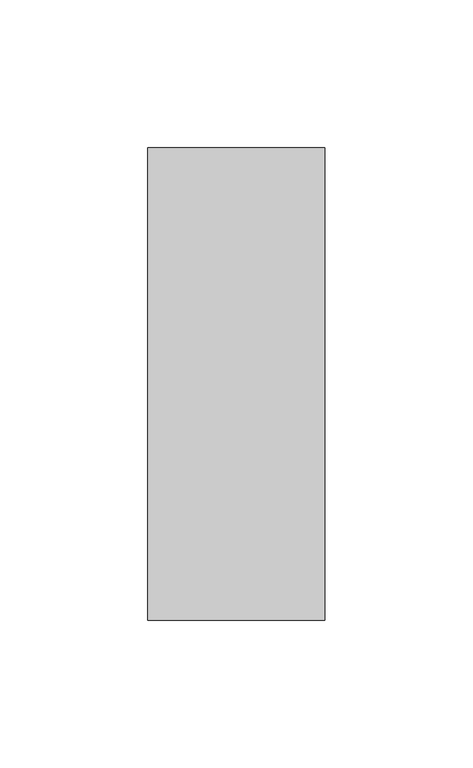
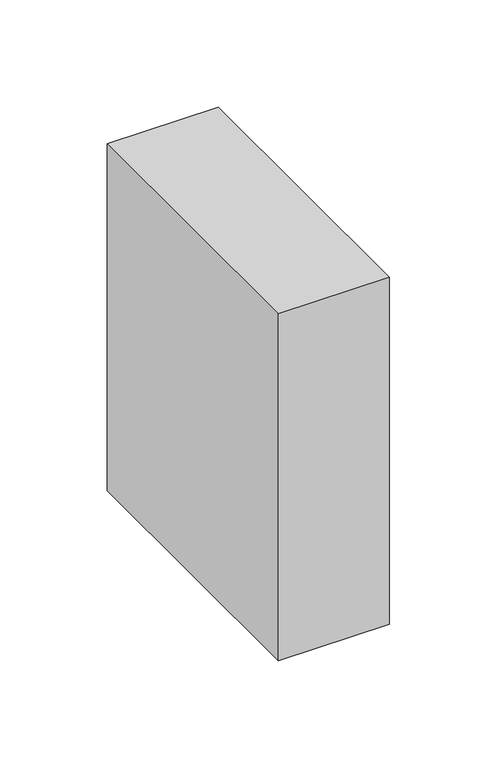
"""IFC4 building model written with IfcOpenShell, lengths in millimetres: column geometry, Madeira de lei-Coluna : Pontalete 6X16cm."""

import ifcopenshell
import ifcopenshell.guid

model = None  # the IFC model being written
_history = None  # IfcOwnerHistory: only IFC2X3 demands one
_inside = {}  # id of a spatial element -> (the spatial element, [elements in it])
_under = {}  # id of a project, library or spatial element -> (it, [spatial elements below it])
_declared = {}  # id of a project -> (the project, [libraries it declares])
_typed = {}  # id of a type object -> (the type object, [elements of that type])
_made_of = {}  # id of a material, layer set ... -> (it, [elements and type objects made of it])


def new_model(schema):
    """Start an empty IFC model of exactly this schema.

    Asked for "IFC4X3", IfcOpenShell would pick the latest addendum, in which some entities
    have other attributes; the version numbers below select the first issue.
    IFC2X3 requires an IfcOwnerHistory on every rooted entity: one is made here for all.
    """
    global model, _history
    if schema == "IFC4X3":
        model = ifcopenshell.file(schema_version=(4, 3, 0, 0))
    else:
        model = ifcopenshell.file(schema=schema)
    _inside.clear()
    _under.clear()
    _declared.clear()
    _typed.clear()
    _made_of.clear()
    _history = None
    if model.schema == "IFC2X3":
        org = make("IfcOrganization", Name="unknown")
        user = make(
            "IfcPersonAndOrganization",
            ThePerson=make("IfcPerson", FamilyName="unknown"),
            TheOrganization=org,
        )
        app = make(
            "IfcApplication",
            ApplicationDeveloper=org,
            Version="unknown",
            ApplicationFullName="unknown",
            ApplicationIdentifier="unknown",
        )
        _history = make(
            "IfcOwnerHistory",
            OwningUser=user,
            OwningApplication=app,
            ChangeAction="ADDED",
            CreationDate=0,
        )
    return model


def make(cls, **values):
    """One entity of the class cls with the attributes given. An attribute that is None is left unset."""
    return model.create_entity(
        cls, **{name: value for name, value in values.items() if value is not None}
    )


def rooted(cls, **values):
    """An entity with a GlobalId (a new one), such as an element, a storey or a relation."""
    return make(cls, GlobalId=ifcopenshell.guid.new(), OwnerHistory=_history, **values)


def si_unit(unit_type, name, prefix=None):
    """IfcSIUnit, for example si_unit("LENGTHUNIT", "METRE", prefix="MILLI")."""
    return make("IfcSIUnit", UnitType=unit_type, Prefix=prefix, Name=name)


def assignment(units):
    """IfcUnitAssignment: the units of a project."""
    return None if units is None else make("IfcUnitAssignment", Units=units)


def point(xyz):
    """IfcCartesianPoint."""
    return None if xyz is None else make("IfcCartesianPoint", Coordinates=xyz)


def direction(xyz):
    """IfcDirection."""
    return None if xyz is None else make("IfcDirection", DirectionRatios=xyz)


def frame(location, z_axis=None, x_axis=None):
    """IfcAxis2Placement3D, a coordinate frame: its origin and axes. An axis left out is left unset."""
    return make(
        "IfcAxis2Placement3D",
        Location=point(location),
        Axis=direction(z_axis),
        RefDirection=direction(x_axis),
    )


def origin():
    """The frame at (0, 0, 0) with its axes left unset."""
    return frame((0.0, 0.0, 0.0))


def place(relative_to, where):
    """IfcLocalPlacement: puts the frame where relative to a parent placement (None: the world)."""
    return make(
        "IfcLocalPlacement", PlacementRelTo=relative_to, RelativePlacement=where
    )


def context(
    kind, dimensions, precision=None, world=None, true_north=None, identifier=None
):
    """IfcGeometricRepresentationContext, for example the 3D "Model" context."""
    return make(
        "IfcGeometricRepresentationContext",
        ContextIdentifier=identifier,
        ContextType=kind,
        CoordinateSpaceDimension=dimensions,
        Precision=precision,
        WorldCoordinateSystem=world,
        TrueNorth=true_north,
    )


def project(units=None, contexts=None):
    """IfcProject with its units and contexts."""
    return rooted(
        "IfcProject",
        Name="project",
        RepresentationContexts=contexts,
        UnitsInContext=assignment(units),
    )


def spatial(cls, under=None, at=None, **own):
    """A site, building, storey or space (cls), placed at a placement, below another one or the project."""
    s = rooted(cls, ObjectPlacement=at, **own)
    if under is not None:
        _under.setdefault(under.id(), (under, []))[1].append(s)
    return s


def polyline(points):
    """IfcPolyline through the points."""
    return make("IfcPolyline", Points=[point(p) for p in points])


def outline(outer, holes=None, kind="AREA"):
    """IfcArbitraryClosedProfileDef: a profile drawn as a closed curve; with holes, ...WithVoids."""
    if holes is None:
        return make("IfcArbitraryClosedProfileDef", ProfileType=kind, OuterCurve=outer)
    return make(
        "IfcArbitraryProfileDefWithVoids",
        ProfileType=kind,
        OuterCurve=outer,
        InnerCurves=holes,
    )


def extrude(swept, where, along, depth):
    """IfcExtrudedAreaSolid: the profile swept, set in the frame where, extruded along a direction by depth."""
    return make(
        "IfcExtrudedAreaSolid",
        SweptArea=swept,
        Position=where,
        ExtrudedDirection=direction(along),
        Depth=depth,
    )


def shape(context_of_items, identifier, shape_type, items):
    """IfcShapeRepresentation: the items that make up one representation, for example the "Body"."""
    return make(
        "IfcShapeRepresentation",
        ContextOfItems=context_of_items,
        RepresentationIdentifier=identifier,
        RepresentationType=shape_type,
        Items=items,
    )


def source(mapping_origin, context_of_items, identifier, shape_type, items):
    """IfcRepresentationMap: a shape defined once, which mapped items show again and again."""
    return make(
        "IfcRepresentationMap",
        MappingOrigin=mapping_origin,
        MappedRepresentation=shape(context_of_items, identifier, shape_type, items),
    )


def transform(
    local_origin,
    x_axis=None,
    y_axis=None,
    z_axis=None,
    scale=None,
    scale2=None,
    scale3=None,
    uniform=True,
):
    """IfcCartesianTransformationOperator3D, or its non-uniform kind. x_axis, y_axis, z_axis: its Axis1, 2, 3."""
    if uniform:
        return make(
            "IfcCartesianTransformationOperator3D",
            Axis1=direction(x_axis),
            Axis2=direction(y_axis),
            LocalOrigin=point(local_origin),
            Scale=scale,
            Axis3=direction(z_axis),
        )
    return make(
        "IfcCartesianTransformationOperator3DnonUniform",
        Axis1=direction(x_axis),
        Axis2=direction(y_axis),
        LocalOrigin=point(local_origin),
        Scale=scale,
        Axis3=direction(z_axis),
        Scale2=scale2,
        Scale3=scale3,
    )


def mapped(mapping_source, mapping_target):
    """IfcMappedItem: shows the shape of a source again, moved by a transform."""
    return make(
        "IfcMappedItem", MappingSource=mapping_source, MappingTarget=mapping_target
    )


def made_of(thing, what):
    """Note that an element or type object is made of a material, layer set ...; save() writes the relation."""
    if what is not None:
        _made_of.setdefault(what.id(), (what, []))[1].append(thing)
    return thing


def element(
    cls,
    number,
    at=None,
    inside=None,
    cuts=None,
    type_object=None,
    material=None,
    context=None,
    identifier="Body",
    shape_type=None,
    held_by="IfcProductDefinitionShape",
    body=None,
    shapes=None,
    **own,
):
    """One element of the class cls, such as IfcWall. Its Tag is "e" and its number.

    at: its placement. inside: the storey or other place that contains it. cuts: it is an
    opening in that element (IfcRelVoidsElement). A single representation is given by context,
    identifier, shape_type and body (its items); several are given by shapes. held_by: the class
    of the entity that holds the representations. save() writes the other relations.
    """
    e = rooted(cls, Tag="e%d" % number, ObjectPlacement=at, **own)
    if body is not None:
        shapes = [shape(context, identifier, shape_type, body)]
    if shapes is not None:
        e.Representation = make(held_by, Representations=shapes)
    if inside is not None:
        _inside.setdefault(inside.id(), (inside, []))[1].append(e)
    if cuts is not None:
        rooted(
            "IfcRelVoidsElement", RelatingBuildingElement=cuts, RelatedOpeningElement=e
        )
    if type_object is not None:
        _typed.setdefault(type_object.id(), (type_object, []))[1].append(e)
    return made_of(e, material)


def aggregate(whole, parts):
    """IfcRelAggregates: a whole, such as a stair, and the parts it consists of."""
    return rooted("IfcRelAggregates", RelatingObject=whole, RelatedObjects=parts)


def save(model, path):
    """Write the relations noted so far, then the file.

    IfcRelAggregates (storeys below a building ...), IfcRelContainedInSpatialStructure (elements
    in a storey), IfcRelDefinesByType, IfcRelAssociatesMaterial and IfcRelDeclares: one each for
    every whole, place, type object, material and project.
    """
    for whole, parts in _under.values():
        aggregate(whole, parts)
    for where, things in _inside.values():
        rooted(
            "IfcRelContainedInSpatialStructure",
            RelatedElements=things,
            RelatingStructure=where,
        )
    for kind, things in _typed.values():
        rooted("IfcRelDefinesByType", RelatedObjects=things, RelatingType=kind)
    for what, things in _made_of.values():
        rooted("IfcRelAssociatesMaterial", RelatedObjects=things, RelatingMaterial=what)
    for by, libraries in _declared.values():
        rooted("IfcRelDeclares", RelatingContext=by, RelatedDefinitions=libraries)
    model.write(path)


def column_35730ad5(model_context):
    return source(origin(), model_context, "Body", "SweptSolid", [
        extrude(outline(polyline([(30.0, 80.0), (30.0, -80.0), (-30.0, -80.0), (-30.0, 80.0), (30.0, 80.0)])), frame((0.0, 0.0, 3110.0), z_axis=(0.0, 0.0, 1.0), x_axis=(1.0, 0.0, 0.0)), (0.0, 0.0, 1.0), 197.9),
    ])


if __name__ == "__main__":
    model = new_model("IFC4")
    model_context = context("Model", 3, world=origin())
    ifc_project = project(units=[si_unit("LENGTHUNIT", "METRE", prefix="MILLI")], contexts=[model_context])
    site = spatial("IfcSite", under=ifc_project)
    building = spatial("IfcBuilding", under=site)
    placement = place(None, origin())
    column_shape = column_35730ad5(model_context)
    element("IfcColumn", 1, ObjectType="Madeira de lei-Coluna : Pontalete 6X16cm", at=placement, inside=building, context=model_context, shape_type="MappedRepresentation", body=[
        mapped(column_shape, transform((0.0, 0.0, 0.0), x_axis=(1.0, 0.0, 0.0), y_axis=(0.0, 1.0, 0.0), z_axis=(0.0, 0.0, 1.0))),
    ])
    save(model, "model.ifc")

# Revit data of these elements
# Type "Madeira de lei-Coluna : Pontalete 6X16cm"
#   A = 0.01952 m²
#   b = 0.06 m
#   d = 0.16 m
#   Structural Material [instance default] = none
#   Assembly Code = ""
# Element 1 (IfcColumn, "Madeira de lei-Coluna : Pontalete 6X16cm")
#   Structural Material = .MADEIRAMENTO
#   Materials on its faces: ".MADEIRAMENTO"
# Materials
#   ".MADEIRAMENTO": class ".CC_MADEIRAS", colour RGB 212 179 113, transparency 0, Cost = 0
